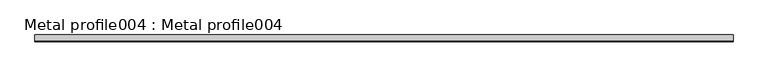
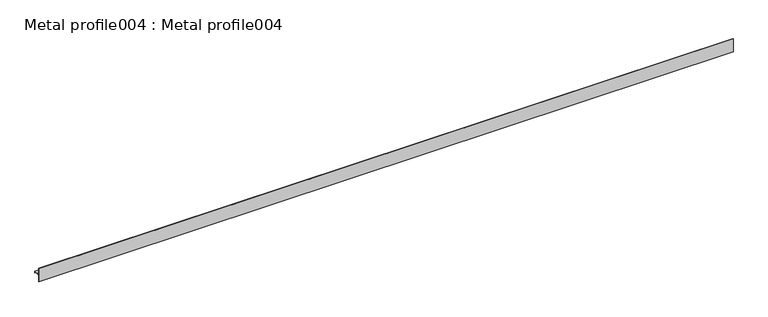
"""IFC4 building model written with IfcOpenShell, lengths in millimetres: proxy geometry, Metal profile004 : Metal profile004."""

from ifc_helpers import new_model, si_unit, frame, origin, place, context, project, spatial, polyline, outline, extrude, source, transform, mapped, element, save


def metal_profile004_metal_profile004_d2acd547(model_context):
    return source(origin(), model_context, "Body", "SweptSolid", [
        extrude(outline(polyline([(10465.4240287, 43386.3870313), (10448.4600807, 43386.3870313), (10448.4600807, 43367.3370312), (10447.1900807, 43367.3370312), (10447.1900807, 43406.7070312), (10448.4600807, 43406.7070312), (10448.4600807, 43387.6570312), (10466.6940287, 43387.6570312), (10466.6940287, 43382.9072312), (10465.4240287, 43382.9072312), (10465.4240287, 43386.3870313)])), frame((3694.2883192, 0.0, 0.0), z_axis=(1.0, 0.0, 0.0), x_axis=(0.0, 1.0, 0.0)), (0.0, 0.0, 1.0), 2000.0),
    ])


if __name__ == "__main__":
    model = new_model("IFC4")
    model_context = context("Model", 3, world=origin())
    ifc_project = project(units=[si_unit("LENGTHUNIT", "METRE", prefix="MILLI")], contexts=[model_context])
    site = spatial("IfcSite", under=ifc_project)
    building = spatial("IfcBuilding", under=site)
    placement = place(None, origin())
    metal_profile004_metal_profile004_shape = metal_profile004_metal_profile004_d2acd547(model_context)
    element("IfcBuildingElementProxy", 1, Name="Metal profile004 : Metal profile004", ObjectType="Metal profile004 : Metal profile004", at=placement, inside=building, context=model_context, shape_type="MappedRepresentation", body=[
        mapped(metal_profile004_metal_profile004_shape, transform((0.0, 0.0, 0.0), x_axis=(1.0, 0.0, 0.0), y_axis=(0.0, 1.0, 0.0), z_axis=(0.0, 0.0, 1.0))),
    ])
    save(model, "model.ifc")

# Revit data of these elements
# Type "Metal profile004 : Metal profile004"
#   NameOverride = "Metal profile004"
# Element 1 (IfcBuildingElementProxy, "Metal profile004 : Metal profile004")
#   Materials on its faces: "16 GA. COPPER VENTED T REVEAL BEAD"
# Materials
#   "16 GA. COPPER VENTED T REVEAL BEAD": class "Unassigned", colour RGB 255 227 10, transparency 0
